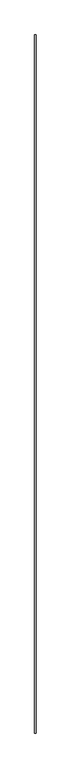
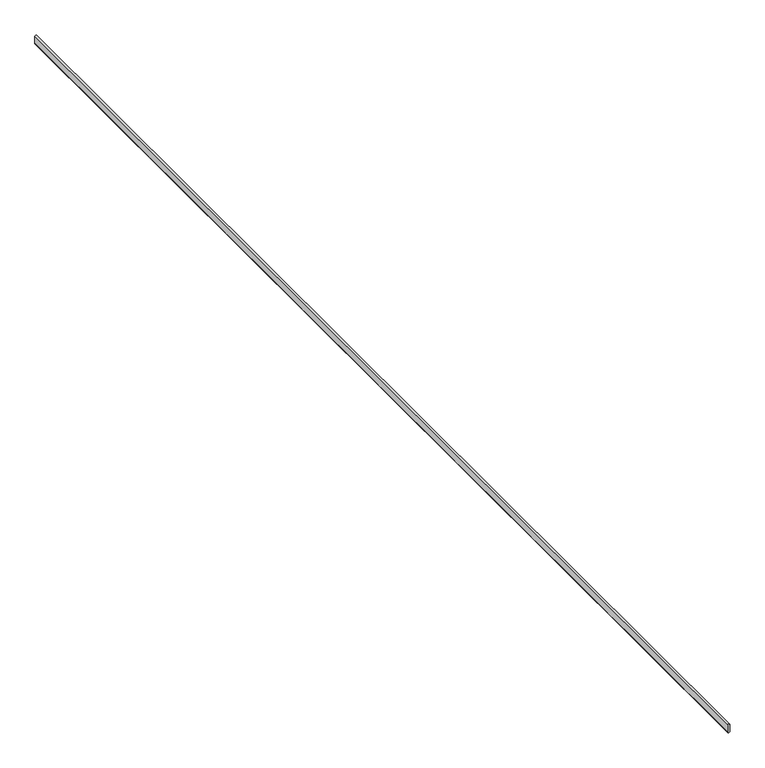
"""IFC4 building model written with IfcOpenShell, lengths in millimetres: proxy geometry, Joint020 15070 : Joint020 15070."""

from ifc_helpers import new_model, si_unit, point, frame, frame_2d, origin, place, context, project, spatial, polyline, circle_curve, trimmed, segment, composite_curve, outline, extrude, source, transform, mapped, element, save


def generic_models_a2196c3a(model_context):
    return source(origin(), model_context, "Body", "SweptSolid", [
        extrude(outline(composite_curve([segment(polyline([(42123.2804083, -2456.7369768), (42111.2057013, -2456.7369768)]), True, "CONTINUOUS"), segment(trimmed(circle_curve(frame_2d((42111.2057013, -2454.9713518)), 1.765625), [point((42111.2057013, -2456.7369768))], [point((42111.2057013, -2453.2057268))], False, "CARTESIAN"), True, "CONTINUOUS"), segment(polyline([(42111.2057013, -2453.2057268), (42123.2804083, -2453.2057268)]), True, "CONTINUOUS"), segment(trimmed(circle_curve(frame_2d((42123.2804083, -2454.9713518)), 1.765625), [point((42123.2804083, -2453.2057268))], [point((42123.2804083, -2456.7369768))], False, "CARTESIAN"), True, "CONTINUOUS")], self_intersect=False)), frame((0.0, -1052.8906574, 0.0), z_axis=(0.0, 1.0, 0.0), x_axis=(0.0, 0.0, 1.0)), (0.0, 0.0, 1.0), 2000.0),
    ])


if __name__ == "__main__":
    model = new_model("IFC4")
    model_context = context("Model", 3, world=origin())
    ifc_project = project(units=[si_unit("LENGTHUNIT", "METRE", prefix="MILLI")], contexts=[model_context])
    site = spatial("IfcSite", under=ifc_project)
    building = spatial("IfcBuilding", under=site)
    placement = place(None, origin())
    generic_models_shape = generic_models_a2196c3a(model_context)
    element("IfcBuildingElementProxy", 1, Name="Joint020 15070 : Joint020 15070", ObjectType="Joint020 15070 : Joint020 15070", at=placement, inside=building, context=model_context, shape_type="MappedRepresentation", body=[
        mapped(generic_models_shape, transform((0.0, 0.0, 0.0), x_axis=(1.0, 0.0, 0.0), y_axis=(0.0, 1.0, 0.0), z_axis=(0.0, 0.0, 1.0))),
    ])
    save(model, "model.ifc")

# Revit data of these elements
# Type "Joint020 15070 : Joint020 15070"
#   NameOverride = "Joint020"
# Element 1 (IfcBuildingElementProxy, "Joint020 15070 : Joint020 15070")
#   Materials on its faces: "SEALANT"
# Materials
#   "SEALANT": class "Unassigned", colour RGB 142 225 148, transparency 0
